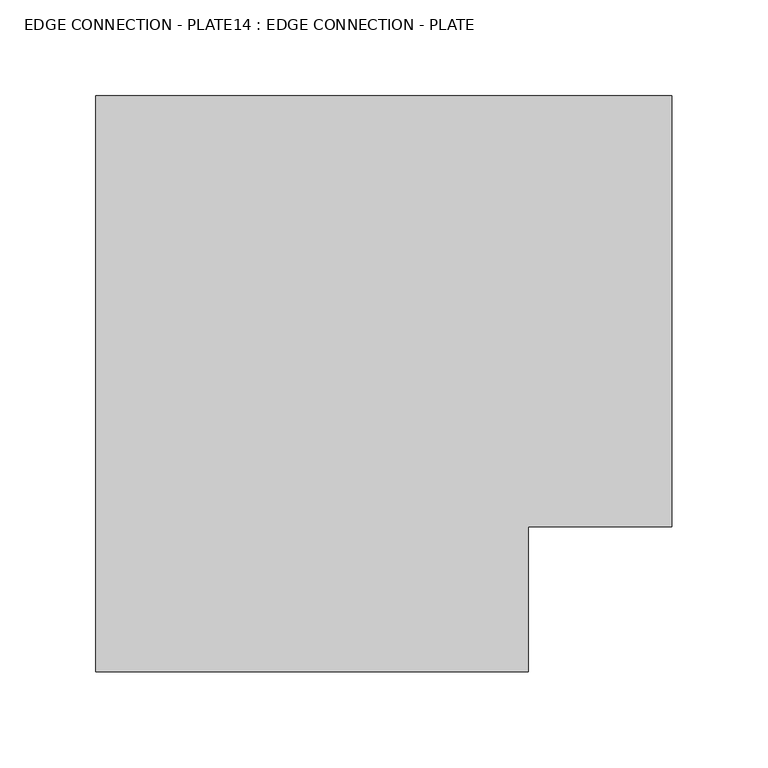
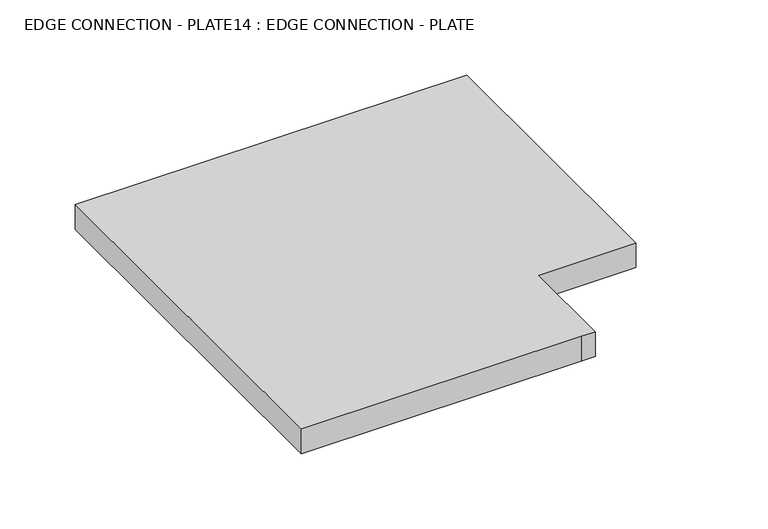
"""IFC4 building model written with IfcOpenShell, lengths in millimetres: fastener geometry, EDGE CONNECTION - PLATE14 : EDGE CONNECTION - PLATE."""

from ifc_helpers import new_model, si_unit, frame, origin, place, context, project, spatial, polyline, outline, extrude, source, transform, mapped, element, save


def edge_connection_plate14_edge_connection_plate_7b59ff89(model_context):
    return source(origin(), model_context, "Body", "SweptSolid", [
        extrude(outline(polyline([(300.0, 25499.5208589), (300.0, 25285.0508589), (300.0, 25275.0508589), (225.138, 25275.0508589), (225.138, 25199.5208589), (215.138, 25199.5208589), (0.0, 25199.5208589), (0.0, 25499.5208589), (300.0, 25499.5208589)])), frame((0.0, 0.0, 200.0), z_axis=(0.0, 0.0, 1.0), x_axis=(1.0, 0.0, 0.0)), (0.0, 0.0, 1.0), 20.0),
    ])


if __name__ == "__main__":
    model = new_model("IFC4")
    model_context = context("Model", 3, world=origin())
    ifc_project = project(units=[si_unit("LENGTHUNIT", "METRE", prefix="MILLI")], contexts=[model_context])
    site = spatial("IfcSite", under=ifc_project)
    building = spatial("IfcBuilding", under=site)
    placement = place(None, origin())
    edge_connection_plate14_edge_connection_plate_shape = edge_connection_plate14_edge_connection_plate_7b59ff89(model_context)
    element("IfcFastener", 1, ObjectType="EDGE CONNECTION - PLATE14 : EDGE CONNECTION - PLATE", at=placement, inside=building, context=model_context, shape_type="MappedRepresentation", body=[
        mapped(edge_connection_plate14_edge_connection_plate_shape, transform((0.0, 0.0, 0.0), x_axis=(1.0, 0.0, 0.0), y_axis=(0.0, 1.0, 0.0), z_axis=(0.0, 0.0, 1.0))),
    ])
    save(model, "model.ifc")
